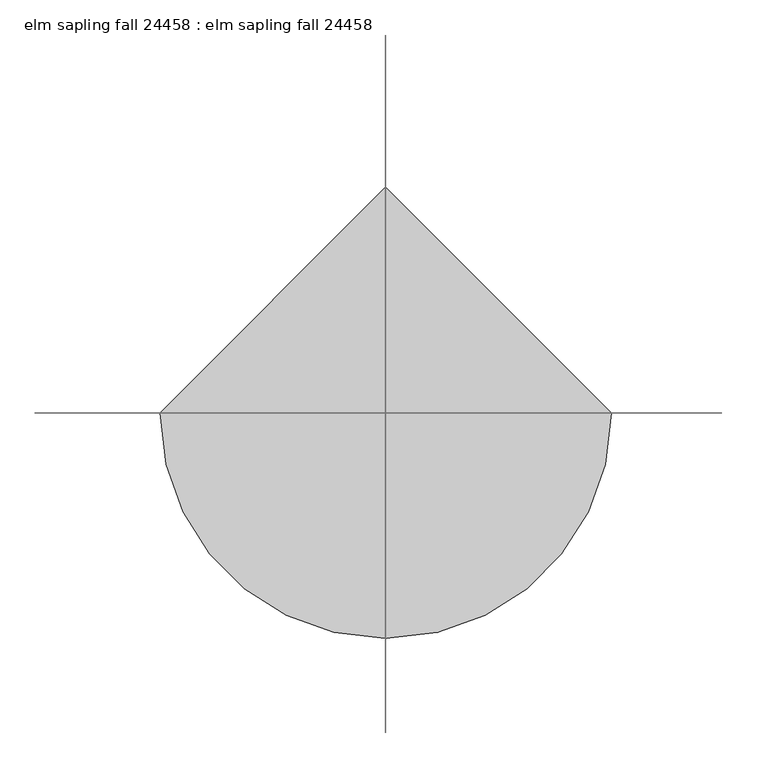
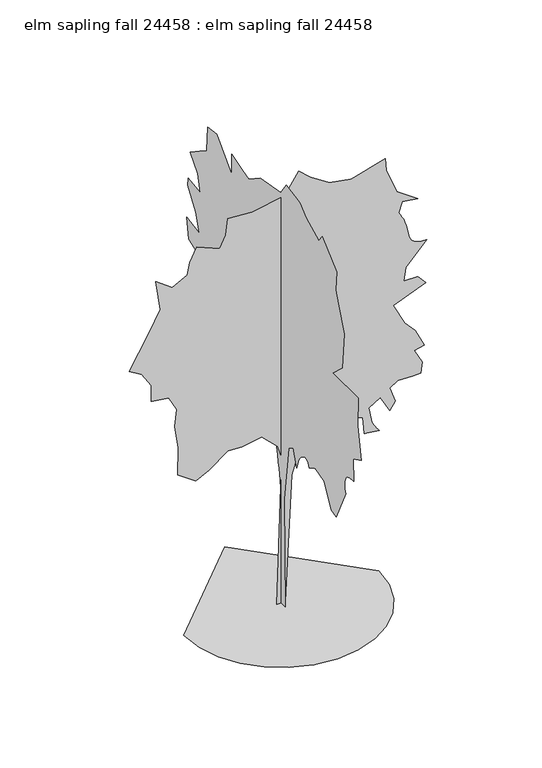
"""IFC4 building model written with IfcOpenShell, lengths in millimetres: proxy geometry, elm sapling fall 24458 : elm sapling fall 24458."""

from ifc_helpers import new_model, si_unit, origin, place, context, project, spatial, triangles, source, transform, mapped, element, save


def elm_sapling_fall_24458_elm_sapling_fall_24458_31049f9d(model_context):
    return source(origin(), model_context, "Body", "Tessellation", [
        triangles([(0.0025148, -47.6280294, 0.2352123), (0.0025387, -35.8607222, 765.0426195), (0.0025449, -88.8133471, 1159.2453747), (0.0025404, -141.765729, 1194.5462723), (0.0025326, -182.9510422, 1076.8757658), (0.0025327, -186.8448634, 1094.5084105), (0.0025328, -191.4077208, 1112.0394625), (0.0025327, -197.3083962, 1129.3648584), (0.0025324, -205.2159077, 1146.3803169), (0.0025318, -215.7998365, 1162.9842453), (0.0025308, -229.7284377, 1179.0751236), (0.0025294, -247.6707291, 1194.5462723), (0.0025278, -266.1283961, 1205.729892), (0.0025263, -281.497934, 1209.8142357), (0.0025249, -294.2944458, 1207.9777925), (0.0025236, -305.0310179, 1201.4093708), (0.0025223, -314.2258055, 1191.2874596), (0.0025211, -322.3919131, 1178.8007944), (0.0025199, -330.0423909, 1165.1280098), (0.0025138, -400.6441861, 1206.314086), (0.0025019, -506.5494587, 1176.8958235), (0.0024887, -588.9190676, 1023.921876), (0.0024827, -641.8729574, 1006.2714272), (0.0024778, -753.6609015, 1235.7324211), (0.0024787, -749.955023, 1252.1128166), (0.0024795, -746.7140144, 1268.4424885), (0.0024803, -744.3975134, 1284.6705677), (0.0024808, -743.4703897, 1300.7435692), (0.0024812, -744.3975134, 1316.61106), (0.0024813, -747.6410654, 1332.2192642), (0.0024812, -753.6609015, 1347.5202198), (0.0024806, -762.4264275, 1360.5910789), (0.0024798, -773.3535221, 1369.9586758), (0.0024786, -786.0814516, 1376.2348915), (0.0024773, -800.2495548, 1380.0423626), (0.0024757, -815.4997141, 1381.9982025), (0.0024741, -831.4686522, 1382.7195248), (0.0024724, -847.798324, 1382.8211174), (0.0024777, -841.9156889, 1541.6803162), (0.0024693, -936.0531115, 1588.7491001), (0.0024803, -894.8670353, 1812.3248428), (0.0024856, -900.7522139, 2012.3675743), (0.0025163, -606.5695527, 2012.3675743), (0.0025083, -712.4748253, 2112.3901028), (0.0025135, -736.0104527, 2371.2693592), (0.002525, -671.2912199, 2530.1260872), (0.0025315, -635.9877789, 2624.2508652), (0.0025343, -647.7555925, 2759.5818489), (0.002556, -483.0163748, 2912.5661156), (0.0025587, -441.8302986, 2859.6071388), (0.0025762, -294.7389499, 2930.2191078), (0.0025861, -218.2529753, 2994.9381226), (0.0026035, -59.3955888, 3024.3514435), (0.0026075, 5.324168, 2930.2191078), (0.0026314, 246.5521201, 2889.0201691), (0.0026429, 381.8761456, 2800.7807877), (0.0026508, 452.4779408, 2818.4337799), (0.0026649, 576.0336622, 2859.6071388), (0.0026605, 576.0336622, 2712.5158264), (0.0026844, 752.5433098, 2894.9131233), (0.0026951, 858.4460026, 2883.1527946), (0.0026932, 864.3311811, 2800.7807877), (0.0026911, 870.2138163, 2706.6228722), (0.0026981, 952.5859686, 2653.6894753), (0.0027074, 1064.37384, 2577.184552), (0.0026953, 976.1190525, 2477.172052), (0.0026887, 946.70079, 2359.5016182), (0.0027039, 1087.9069965, 2377.1519943), (0.002703, 1093.7921751, 2324.2007206), (0.0026891, 999.6546799, 2188.8771492), (0.0026811, 958.4686037, 2065.3214642), (0.0026972, 1105.5599888, 2088.8544754), (0.0026905, 1082.0243614, 1947.6484142), (0.0026803, 993.7695013, 1912.3475166), (0.002667, 870.2138163, 1900.5796303), (0.0026603, 840.7955538, 1777.0239452), (0.0026451, 740.7754961, 1618.1673626), (0.0026388, 681.9388985, 1612.2821114), (0.00263, 611.3345598, 1565.2134727), (0.0026307, 652.520636, 1441.6576424), (0.0026227, 599.5692896, 1359.2881062), (0.00262, 605.4519247, 1247.5001621), (0.0026253, 681.9388985, 1159.2453747), (0.0026163, 605.4519247, 1123.9444771), (0.0026168, 570.1510271, 1265.1506836), (0.0026099, 505.431867, 1259.2654324), (0.002601, 440.7101272, 1188.6636372), (0.0025991, 452.4779408, 1082.7584009), (0.0025979, 470.128426, 982.7383432), (0.0025922, 399.5265944, 1035.6896896), (0.0025979, 411.2944081, 1188.6636372), (0.0025945, 358.3405183, 1259.2654324), (0.0025769, 187.7160856, 1265.1506836), (0.0025618, 70.0440258, 1171.0131884), (0.0025547, 40.7118636, 1033.1496557), (0.0025524, 31.8950213, 989.3575613), (0.0025503, 23.9014662, 947.417098), (0.0025484, 16.9372463, 907.7930632), (0.0025468, 11.2080504, 870.9478558), (0.0025448, 7.7087955, 817.6358482), (0.0025422, 6.9883753, 731.9032179), (0.002539, 8.5836472, 619.1552307), (0.0025228, 28.8589602, 0.2352169), (-30.3527349, -0.0131541, 0.0), (5.2258449, -0.0132761, 1037.8131065), (-24.4228779, -0.0132836, 1126.7587675), (-131.1584368, -0.0132999, 1233.4946217), (-267.5431716, -0.0132894, 1209.7760839), (-362.4197388, -0.0132959, 1215.7045012), (-486.9432063, -0.0132786, 1120.830423), (-575.8889036, -0.0132799, 1073.3908768), (-700.4148783, -0.0132933, 1162.3365377), (-694.4839903, -0.0133135, 1352.0897083), (-718.2049988, -0.0133287, 1512.1934532), (-706.3432228, -0.0133418, 1630.7885399), (-759.7111862, -0.0133608, 1731.5935787), (-878.3062729, -0.0133555, 1749.3836266), (-878.3062729, -0.0133673, 1862.0478252), (-943.5333961, -0.0133855, 1962.8528641), (-1026.5507853, -0.0133861, 2016.2206821), (-896.0963934, -0.0134174, 2241.5516956), (-819.0099649, -0.0134368, 2383.8652473), (-848.6593906, -0.0134573, 2597.3266365), (-735.9926485, -0.0134554, 2514.32211), (-635.1876823, -0.0134554, 2567.6848412), (-617.3975618, -0.0134651, 2650.7175636), (-569.9605227, -0.0134778, 2745.5864822), (-415.7876658, -0.0134686, 2680.359359), (-374.2790076, -0.0134798, 2763.3665016), (-362.4197388, -0.0134922, 2876.0407288), (-196.3856146, -0.0134893, 2864.1789528), (23.0151082, -0.0134951, 2905.6825241), (117.8912597, -0.0135156, 3047.9988373), (194.9779425, -0.0135012, 2976.8534706), (325.4322799, -0.0135003, 2893.8207481), (473.6767922, -0.0134945, 2864.1789528), (704.9361139, -0.0135035, 2929.4063667), (710.8670019, -0.0134952, 2846.3989334), (782.0225424, -0.0134693, 2668.497583), (924.3360941, -0.0134557, 2567.6848412), (817.6027834, -0.0134628, 2585.4904404), (793.8817749, -0.013454, 2514.32211), (805.2762102, -0.0134526, 2495.147699), (816.4090336, -0.0134512, 2475.3026894), (827.0236473, -0.0134381, 2454.1063087), (836.8610556, -0.0134362, 2430.8882492), (845.6596464, -0.0134341, 2404.9751507), (853.1628222, -0.0134315, 2375.6890022), (859.1089708, -0.0134283, 2342.3590599), (866.7848104, -0.0134256, 2311.4472839), (879.1291878, -0.0134239, 2288.9379021), (895.3623539, -0.0134233, 2273.4311451), (914.706958, -0.0134234, 2263.525209), (936.3884108, -0.0134241, 2257.8203247), (959.6218037, -0.0134252, 2254.9171589), (983.6349455, -0.0134149, 2253.4108555), (841.3213211, -0.0134025, 2105.1688866), (829.4620886, -0.0133919, 2010.2924103), (924.3386375, -0.013386, 2010.2924103), (977.7040575, -0.013383, 1950.9935589), (758.3040047, -0.0133722, 1862.0478252), (835.3904331, -0.0133492, 1707.8749683), (906.548517, -0.0133454, 1630.7885399), (965.8447523, -0.0133359, 1506.2625652), (900.6176291, -0.0133302, 1488.4749882), (953.9855198, -0.0133112, 1387.6674786), (942.1262873, -0.0133031, 1316.5119381), (888.7583239, -0.0133109, 1310.5810501), (787.9534304, -0.0133055, 1316.5119381), (734.585467, -0.0132986, 1280.9316971), (770.1632372, -0.0132896, 1174.1983864), (734.585467, -0.0132819, 1120.830423), (669.3583437, -0.0133014, 1233.4946217), (592.2718789, -0.0132918, 1186.0576189), (610.0594923, -0.0132836, 1097.1094145), (613.6383436, -0.0132823, 1082.2071991), (619.0840868, -0.0132811, 1067.9273294), (626.086857, -0.0132801, 1054.1681402), (634.3317026, -0.0132792, 1040.8204811), (643.5138456, -0.0132784, 1027.7851576), (653.3156456, -0.013266, 1014.9581789), (663.427383, -0.0132653, 1002.2353363), (562.6224895, -0.0132721, 1014.0945688), (550.7632207, -0.0132838, 1132.6896555), (479.6051368, -0.0132936, 1156.4081932), (408.4496326, -0.0132955, 1215.7045012), (289.8545278, -0.0133007, 1221.6353165), (289.8545278, -0.013273, 1067.4625322), (224.6268414, -0.0132801, 1061.5316442), (242.4159808, -0.0132953, 1197.9168514), (147.5399042, -0.0132841, 1144.5489607), (70.4532214, -0.013253, 889.5685942), (28.944813, -0.0131461, 0.1174198), (-660.3032278, 1.02e-05, 0.2309946), (-642.8483339, -151.2980869, 0.2309847), (-593.1329455, -290.2406053, 0.2309735), (-515.139741, -412.8488917, 0.2309614), (-412.8488917, -515.139741, 0.2309492), (-290.2406053, -593.1329455, 0.2309372), (-151.2978325, -642.8483339, 0.230926), (2.89e-05, -660.3032278, 0.2309159), (151.2980869, -642.8483339, 0.230908), (290.2406053, -593.1329455, 0.2309027), (412.8488917, -515.139741, 0.2309001), (515.139741, -412.8488917, 0.2309001), (593.1329455, -290.2406053, 0.2309027), (642.8483339, -151.2978325, 0.230908), (660.3032278, 5.88e-05, 0.2309159), (-8.66e-05, 660.3032278, 0.2309946)], [[4, 5, 6], [4, 6, 7], [88, 89, 90], [88, 90, 91], [87, 88, 91], [4, 7, 8], [4, 8, 9], [71, 72, 73], [71, 73, 74], [57, 58, 59], [82, 83, 84], [82, 84, 85], [81, 82, 85], [71, 74, 75], [64, 65, 66], [48, 49, 50], [4, 9, 10], [102, 103, 1], [102, 1, 2], [101, 102, 2], [100, 101, 2], [100, 2, 3], [99, 100, 3], [98, 99, 3], [97, 98, 3], [96, 97, 3], [95, 96, 3], [37, 38, 39], [41, 42, 43], [18, 19, 20], [94, 95, 3], [67, 68, 69], [67, 69, 70], [36, 37, 39], [22, 23, 24], [21, 22, 24], [21, 24, 25], [21, 25, 26], [60, 61, 62], [59, 60, 62], [59, 62, 63], [21, 26, 27], [17, 18, 20], [39, 40, 41], [35, 36, 39], [4, 10, 11], [47, 48, 50], [21, 27, 28], [81, 85, 86], [39, 41, 43], [52, 53, 54], [34, 35, 39], [21, 28, 29], [16, 17, 20], [51, 52, 54], [56, 57, 59], [87, 91, 92], [86, 87, 92], [76, 77, 78], [79, 80, 81], [4, 11, 12], [63, 64, 66], [59, 63, 66], [59, 66, 67], [21, 29, 30], [20, 21, 30], [20, 30, 31], [81, 86, 92], [79, 81, 92], [79, 92, 93], [34, 39, 43], [33, 34, 43], [32, 33, 43], [31, 32, 43], [20, 31, 43], [16, 20, 43], [15, 16, 43], [14, 15, 43], [13, 14, 43], [43, 44, 45], [43, 45, 46], [94, 3, 4], [93, 94, 4], [12, 13, 43], [4, 12, 43], [93, 4, 43], [79, 93, 43], [79, 43, 46], [79, 46, 47], [79, 47, 50], [79, 50, 51], [79, 51, 54], [79, 54, 55], [79, 55, 56], [79, 56, 59], [79, 59, 67], [78, 79, 67], [76, 78, 67], [75, 76, 67], [71, 75, 67], [71, 67, 70], [139, 140, 141], [181, 182, 183], [122, 123, 124], [155, 156, 157], [180, 181, 183], [154, 155, 157], [171, 172, 173], [170, 171, 173], [179, 180, 183], [159, 160, 161], [158, 159, 161], [153, 154, 157], [179, 183, 184], [178, 179, 184], [177, 178, 184], [176, 177, 184], [175, 176, 184], [174, 175, 184], [188, 189, 190], [187, 188, 190], [136, 137, 138], [163, 164, 165], [132, 133, 134], [193, 104, 105], [192, 193, 105], [191, 192, 105], [191, 105, 106], [129, 130, 131], [152, 153, 157], [119, 120, 121], [126, 127, 128], [116, 117, 118], [166, 167, 168], [174, 184, 185], [125, 126, 128], [165, 166, 168], [165, 168, 169], [151, 152, 157], [136, 138, 139], [110, 111, 112], [110, 112, 113], [109, 110, 113], [109, 113, 114], [109, 114, 115], [132, 134, 135], [174, 185, 186], [191, 106, 107], [190, 191, 107], [108, 109, 115], [107, 108, 115], [162, 163, 165], [162, 165, 169], [162, 169, 170], [118, 119, 121], [139, 141, 142], [136, 139, 142], [173, 174, 186], [162, 170, 173], [162, 173, 186], [161, 162, 186], [161, 186, 187], [150, 151, 157], [116, 118, 121], [116, 121, 122], [116, 122, 124], [116, 124, 125], [116, 125, 128], [115, 116, 128], [107, 115, 128], [190, 107, 128], [187, 190, 128], [161, 187, 128], [158, 161, 128], [157, 158, 128], [150, 157, 128], [149, 150, 128], [148, 149, 128], [147, 148, 128], [146, 147, 128], [145, 146, 128], [144, 145, 128], [143, 144, 128], [142, 143, 128], [136, 142, 128], [135, 136, 128], [132, 135, 128], [131, 132, 128], [129, 131, 128], [208, 209, 194], [207, 208, 194], [207, 194, 195], [206, 207, 195], [206, 195, 196], [206, 196, 197], [205, 206, 197], [204, 205, 197], [204, 197, 198], [204, 198, 199], [204, 199, 200], [204, 200, 201], [204, 201, 202], [204, 202, 203]], closed=False),
    ])


if __name__ == "__main__":
    model = new_model("IFC4")
    model_context = context("Model", 3, world=origin())
    ifc_project = project(units=[si_unit("LENGTHUNIT", "METRE", prefix="MILLI")], contexts=[model_context])
    site = spatial("IfcSite", under=ifc_project)
    building = spatial("IfcBuilding", under=site)
    placement = place(None, origin())
    elm_sapling_fall_24458_elm_sapling_fall_24458_shape = elm_sapling_fall_24458_elm_sapling_fall_24458_31049f9d(model_context)
    element("IfcBuildingElementProxy", 1, Name="elm sapling fall 24458 : elm sapling fall 24458", ObjectType="elm sapling fall 24458 : elm sapling fall 24458", at=placement, inside=building, context=model_context, shape_type="MappedRepresentation", body=[
        mapped(elm_sapling_fall_24458_elm_sapling_fall_24458_shape, transform((0.0, 0.0, 0.0), x_axis=(1.0, 0.0, 0.0), y_axis=(0.0, 1.0, 0.0), z_axis=(0.0, 0.0, 1.0))),
    ])
    save(model, "model.ifc")

# Revit data of these elements
# Type "elm sapling fall 24458 : elm sapling fall 24458"
#   built-in parameter 1005195 = "RPC-16-FWVN-NVXX-5TD6-C000-ST1L-LVER-AU"
#   Height = 0
